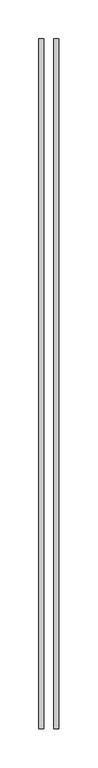
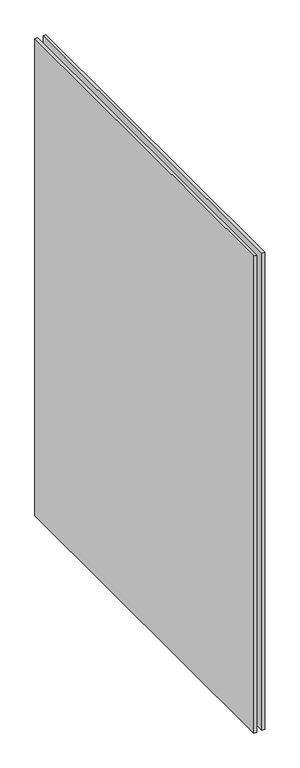
"""IFC4 building model written with IfcOpenShell, lengths in millimetres: proxy geometry, Window glass:Window glass:1:Window glass:1 : Window glass:Window glass:300352:337881:Window glass:1:Window glass:1 : Window glass:Window glass:300352:337881 : Window glass:Window glass:1:Window glass:1 : Window glass:Window glass:300352:337881:2 : Window glass:Window glass:1:Window glass:1 : Window glass:Window glass:300352:337881:Window glass:1:Window glass:1 : Window glass:Window glass:300352:337881 : Window glass:Window glass:1:Window glass:1 : Window glass:Window glass:300352:337881:301362."""

from ifc_helpers import new_model, si_unit, frame, origin, place, context, project, spatial, polyline, outline, extrude, source, transform, mapped, element, save


def generic_models_f31c8460(model_context):
    return source(origin(), model_context, "Body", "SweptSolid", [
        extrude(outline(polyline([(560292.6367239, -573499.7590038), (560292.6367239, -572612.5407192), (560298.9867239, -572612.5407192), (560298.9867239, -573499.7590038), (560292.6367239, -573499.7590038)])), frame((0.0, 0.0, 2479.9705452), z_axis=(0.0, 0.0, 1.0), x_axis=(1.0, 0.0, 0.0)), (0.0, 0.0, 1.0), 1180.5089096),
        extrude(outline(polyline([(560311.6867239, -573499.7590038), (560311.6867239, -572612.5407192), (560318.0367239, -572612.5407192), (560318.0367239, -573499.7590038), (560311.6867239, -573499.7590038)])), frame((0.0, 0.0, 2479.9705452), z_axis=(0.0, 0.0, 1.0), x_axis=(1.0, 0.0, 0.0)), (0.0, 0.0, 1.0), 1180.5089096),
    ])


if __name__ == "__main__":
    model = new_model("IFC4")
    model_context = context("Model", 3, world=origin())
    ifc_project = project(units=[si_unit("LENGTHUNIT", "METRE", prefix="MILLI")], contexts=[model_context])
    site = spatial("IfcSite", under=ifc_project)
    building = spatial("IfcBuilding", under=site)
    placement = place(None, origin())
    generic_models_shape = generic_models_f31c8460(model_context)
    element("IfcBuildingElementProxy", 1, Name="Window glass:Window glass:1:Window glass:1 : Window glass:Window glass:300352:337881:Window glass:1:Window glass:1 : Window glass:Window glass:300352:337881 : Window glass:Window glass:1:Window glass:1 : Window glass:Window glass:300352:337881:2 : Window glass:Window glass:1:Window glass:1 : Window glass:Window glass:300352:337881:Window glass:1:Window glass:1 : Window glass:Window glass:300352:337881 : Window glass:Window glass:1:Window glass:1 : Window glass:Window glass:300352:337881:301362", ObjectType="Window glass:Window glass:1:Window glass:1 : Window glass:Window glass:300352:337881:Window glass:1:Window glass:1 : Window glass:Window glass:300352:337881 : Window glass:Window glass:1:Window glass:1 : Window glass:Window glass:300352:337881:2 : Window glass:Window glass:1:Window glass:1 : Window glass:Window glass:300352:337881:Window glass:1:Window glass:1 : Window glass:Window glass:300352:337881 : Window glass:Window glass:1:Window glass:1 : Window glass:Window glass:300352:337881:301362", at=placement, inside=building, context=model_context, shape_type="MappedRepresentation", body=[
        mapped(generic_models_shape, transform((0.0, 0.0, 0.0), x_axis=(1.0, 0.0, 0.0), y_axis=(0.0, 1.0, 0.0), z_axis=(0.0, 0.0, 1.0))),
    ])
    save(model, "model.ifc")

# Revit data of these elements
# Type "Window glass:Window glass:1:Window glass:1 : Window glass:Window glass:300352:337881:Window glass:1:Window glass:1 : Window glass:Window glass:300352:337881 : Window glass:Window glass:1:Window glass:1 : Window glass:Window glass:300352:337881:2 : Window glass:Window glass:1:Window glass:1 : Window glass:Window glass:300352:337881:Window glass:1:Window glass:1 : Window glass:Window glass:300352:337881 : Window glass:Window glass:1:Window glass:1 : Window glass:Window glass:300352:337881:301362"
#   NameOverride = "Window glass:Window glass:1:Window glass:1 : Window glass:Window glass:300352:337881:Window glass:1:Window glass:1 : Window glass:Window glass:300352:337881 : Window glass:Window glass:1:Window glass:1 : Window glass:Window glass:300352:337881:301362"
#   ObjectTypeOverride = "Window glass:1:Window glass:1 : Window glass:Window glass:300352:337881 : Window glass:Window glass:1:Window glass:1 : Window glass:Window glass:300352:337881"
#   Reference = "Window glass"
#   Tag = "301362"
# Element 1 (IfcBuildingElementProxy, "Window glass:Window glass:1:Window glass:1 : Window glass:Window glass:300352:337881:Window glass:1:Window glass:1 : Window glass:Window glass:300352:337881 : Window glass:Window glass:1:Window glass:1 : Window glass:Window glass:300352:337881:2 : Window glass:Window glass:1:Window glass:1 : Window glass:Window glass:300352:337881:Window glass:1:Window glass:1 : Window glass:Window glass:300352:337881 : Window glass:Window glass:1:Window glass:1 : Window glass:Window glass:300352:337881:301362")
#   Materials on its faces: "INSULATED LOW-E GLAZING (SEE ELEVATIONS FOR U-FACTOR, SHGC, & LT)"
# Materials
#   "INSULATED LOW-E GLAZING (SEE ELEVATIONS FOR U-FACTOR, SHGC, & LT)": class "Unassigned", colour RGB 84 171 255, transparency 0, Cost = 0
